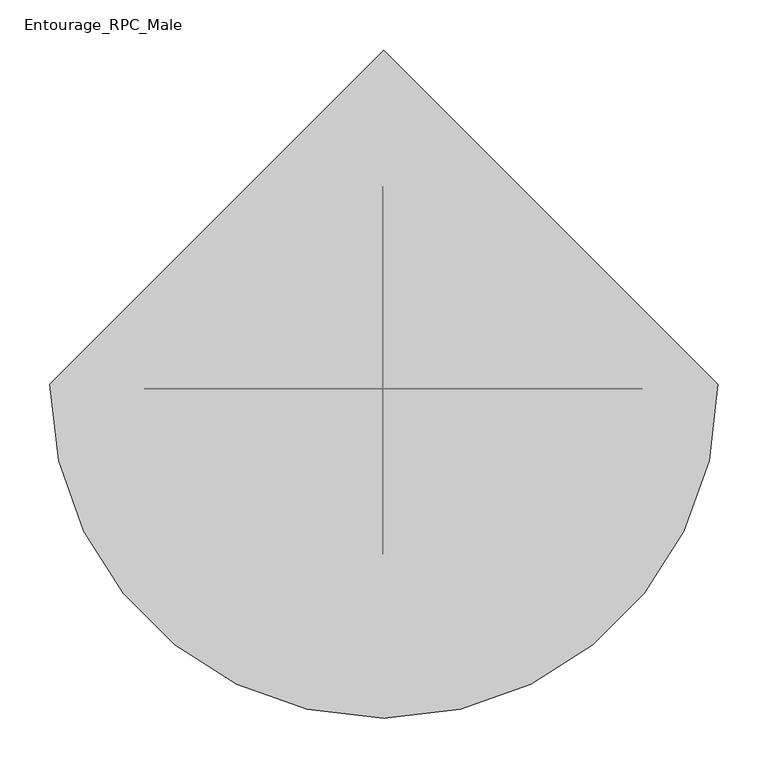
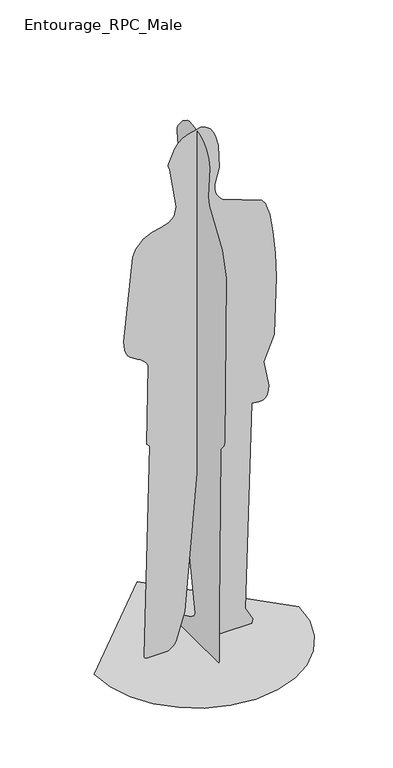
"""IFC4 building model written with IfcOpenShell, lengths in millimetres: proxy geometry, Entourage_RPC_Male : Dwayne."""

from ifc_helpers import new_model, si_unit, origin, place, context, project, spatial, triangles, source, transform, mapped, element, save


def entourage_rpc_male_e00c4429(model_context):
    return source(origin(), model_context, "Body", "Tessellation", [
        triangles([(-180.7519758, -4.45e-05, 5.61e-05), (-184.2427693, -8.8e-06, 2.7953145), (-186.1721755, 1.66e-05, 5.8375002), (-186.8316374, 3.35e-05, 9.127569), (-168.2846227, 8.5e-06, 733.0652109), (-173.8813015, 8.5e-06, 735.2240908), (-177.6698602, 8.1e-06, 740.93319), (-174.1985423, -8.1e-06, 1013.6682867), (-179.591309, -8.8e-06, 1024.1651751), (-188.0395216, -9.6e-06, 1032.7759867), (-198.5267085, -9.9e-06, 1040.1126028), (-210.0363257, -1.03e-05, 1046.7864687), (-221.5520472, -1.07e-05, 1053.4092476), (-232.0572199, -1.1e-05, 1060.5929661), (-240.5353907, -1.14e-05, 1068.9488514), (-245.9518842, -1.21e-05, 1078.9880642), (-249.7386988, -1.29e-05, 1091.9821838), (-252.1552483, -1.4e-05, 1106.9298906), (-253.4607645, -1.47e-05, 1122.8295742), (-224.2188539, -3.16e-05, 1405.054644), (-213.7949444, -3.31e-05, 1430.2019463), (-189.1319694, -3.46e-05, 1456.0842327), (-160.624934, -3.53e-05, 1468.8737137), (-131.9229886, -3.57e-05, 1475.6378357), (-106.6752928, -3.64e-05, 1483.4436092), (-88.5310242, -3.71e-05, 1499.3593529), (-81.1392697, -3.9e-05, 1530.4516411), (-102.942045, -4.71e-05, 1666.4696468), (-107.9472446, -4.78e-05, 1679.2650867), (-108.1474504, -4.82e-05, 1680.5741638), (-107.984815, -4.82e-05, 1682.7587688), (-107.5268306, -4.82e-05, 1685.5190655), (-106.840944, -4.86e-05, 1688.5553627), (-86.6409052, -5.11e-05, 1733.0902897), (-74.2774293, -5.19e-05, 1747.7183212), (-59.5121605, -5.26e-05, 1759.6594528), (-42.363121, -5.33e-05, 1768.7777916), (-0.9855255, -5.37e-05, 1777.9990311), (15.8808757, -5.33e-05, 1772.5528519), (29.1619555, -5.26e-05, 1761.5639877), (39.2640369, -5.19e-05, 1747.0962662), (46.5934632, -5.08e-05, 1731.2140961), (56.009163, -4.89e-05, 1695.7207684), (59.1639487, -4.41e-05, 1618.2087845), (44.4858339, -4.12e-05, 1564.7278919), (44.3096682, -4.05e-05, 1551.1862766), (46.5532813, -3.94e-05, 1537.9279289), (51.2886345, -3.86e-05, 1525.4359589), (58.5876575, -3.83e-05, 1514.1926044), (68.5223164, -3.75e-05, 1504.6808304), (198.4030241, -3.46e-05, 1454.5808361), (210.7095586, -3.38e-05, 1440.8296406), (224.9005892, -3.13e-05, 1397.8447643), (235.5369131, -2.72e-05, 1333.6069702), (242.7580384, -2.28e-05, 1256.1532677), (246.7032373, -1.77e-05, 1173.5211021), (240.2781571, -5.9e-06, 974.9290089), (206.081389, -1.1e-06, 891.6222479), (221.1961823, 4e-06, 805.6633232), (220.4650678, 5.1e-06, 788.6200321), (214.9948893, 6.3e-06, 771.8045614), (210.3552016, 6.6e-06, 765.7300776), (204.1668257, 6.6e-06, 762.0919275), (196.8959759, 7e-06, 760.3982082), (189.0090118, 7e-06, 760.1573799), (180.9721295, 7e-06, 760.8774668), (173.2515615, 6.6e-06, 762.0669291), (166.3135766, 6.6e-06, 763.2339363), (144.8011179, 4.49e-05, 59.4752896), (168.6275342, 4.74e-05, 15.3365843), (166.1985945, -4.45e-05, 5.61e-05), (66.1332089, -4.45e-05, 5.61e-05), (49.8425018, -1.03e-05, 3.9765591), (39.0246256, 1.36e-05, 14.0353), (32.5983009, 2.91e-05, 28.3297116), (-2.7441046, 9.2e-06, 720.0458748), (-54.0725034, 1.03e-05, 117.9433278), (-81.3720135, -2.13e-05, 28.0047427), (-85.5237041, -2.69e-05, 19.9172686), (-91.2433859, -3.27e-05, 12.5691172), (-99.2451413, -3.86e-05, 5.9378887), (-110.2431982, -4.45e-05, 5.61e-05), (-13.8237406, -127.6718764, 9.9621145), (-13.8237974, -127.2617633, 182.0842528), (-13.8237815, -135.2635732, 744.8695776), (-13.8237815, -136.4149928, 748.3460369), (-13.8237815, -139.3954704, 752.5736132), (-13.8237815, -143.4944026, 757.5058702), (-13.8237815, -148.0010861, 763.0962994), (-13.8237815, -152.2049901, 769.2983917), (-13.8237792, -155.3953659, 776.0656385), (-13.8237792, -156.8616281, 783.3516764), (-13.8237622, -165.9465024, 1358.6137287), (-13.8237599, -143.2743216, 1442.0927902), (-13.8237576, -71.1145501, 1552.8585583), (-13.8237576, -64.3401725, 1580.5206779), (-13.8237542, -73.5344014, 1684.7952724), (-13.8237531, -67.2131212, 1712.2161278), (-13.8237531, -55.241223, 1734.9070393), (-13.8237531, -37.9260212, 1752.7537697), (-13.8237531, -15.5748771, 1765.6426632), (-13.8237531, 11.5049084, 1773.4593372), (-13.8237531, 43.0059914, 1776.090136), (-13.8237531, 55.0860226, 1772.9164925), (-13.8237542, 79.7038559, 1756.3218658), (-13.8237554, 107.4896145, 1722.3477768), (-13.8237554, 111.5711695, 1713.01012), (-13.8237554, 112.2229284, 1702.3019073), (-13.8237588, 99.0832235, 1611.9284992), (-13.8237588, 100.6007272, 1597.8206394), (-13.8237599, 96.755177, 1579.0656796), (-13.8237622, 31.1784566, 1488.4592915), (-13.8237735, 125.7984261, 1146.7472277), (-13.8237735, 134.1993577, 1137.675107), (-13.8237747, 184.2799037, 1119.3925747), (-13.8237747, 194.4649651, 1111.9394686), (-13.8237747, 201.1343255, 1100.3801451), (-13.8237769, 203.5508567, 1084.2058416), (-13.8237769, 200.9674025, 1068.9640394), (-13.8237769, 194.2820729, 1055.8707253), (-13.8237769, 184.3928146, 1046.1415226), (-13.8237769, 172.1978105, 1040.992709), (-13.8237769, 158.595007, 1041.6399078), (-13.8237769, 144.48246, 1049.299106), (-13.8237838, 123.0429529, 785.7648285), (-13.823786, 116.906318, 707.2429499), (-13.8237928, 10.2023683, 90.6853168), (-13.823794, 17.983895, 76.1481908), (-13.8237951, 35.4714404, 63.806743), (-13.8238042, 104.5965316, 31.8661463), (-13.8238053, 119.3344402, 20.2173661), (-13.8238076, 122.9915025, 6.7192091), (-13.8238042, 122.0607091, 4.3674998), (-13.8237894, 120.3451706, 2.3141478), (-13.8237724, 119.1853577, 1.4285653), (-13.8237474, 117.8199432, 0.6534771), (-13.8237099, 116.2458387, 5.61e-05), (-13.8237077, -124.501612, 0.0), (-348.4734607, 4.7230039, 0.0001684), (-339.5987117, -72.1961519, 0.0001684), (-314.3237646, -142.8340959, 5.61e-05), (-274.6722241, -205.1669827, 5.61e-05), (-222.6681673, -257.171094, 5.61e-05), (-160.3352533, -296.8225073, 5.61e-05), (-89.6973139, -322.097527, 5.61e-05), (-12.7781649, -330.972276, 5.61e-05), (64.1409886, -322.0975634, 5.61e-05), (134.7789371, -296.8225618, 5.61e-05), (197.1118239, -257.1710577, 5.61e-05), (249.1159897, -205.1670008, 5.61e-05), (288.7673667, -142.8340595, 5.61e-05), (314.0423864, -72.1960974, 0.0001684), (322.9171354, 4.7230331, 0.0001684), (-12.7782239, 340.4182474, 0.0001684)], [[70, 71, 72], [69, 70, 72], [69, 72, 73], [69, 73, 74], [69, 74, 75], [69, 75, 76], [68, 69, 76], [82, 1, 2], [82, 2, 3], [82, 3, 4], [81, 82, 4], [80, 81, 4], [79, 80, 4], [78, 79, 4], [77, 78, 4], [77, 4, 5], [76, 77, 5], [5, 6, 7], [76, 5, 7], [76, 7, 8], [68, 76, 8], [67, 68, 8], [66, 67, 8], [65, 66, 8], [64, 65, 8], [63, 64, 8], [62, 63, 8], [61, 62, 8], [60, 61, 8], [59, 60, 8], [58, 59, 8], [57, 58, 8], [56, 57, 8], [56, 8, 9], [55, 56, 9], [55, 9, 10], [54, 55, 10], [54, 10, 11], [53, 54, 11], [53, 11, 12], [52, 53, 12], [51, 52, 12], [50, 51, 12], [50, 12, 13], [50, 13, 14], [50, 14, 15], [50, 15, 16], [50, 16, 17], [50, 17, 18], [50, 18, 19], [50, 19, 20], [50, 20, 21], [50, 21, 22], [50, 22, 23], [50, 23, 24], [50, 24, 25], [50, 25, 26], [49, 50, 26], [48, 49, 26], [48, 26, 27], [47, 48, 27], [46, 47, 27], [45, 46, 27], [44, 45, 27], [44, 27, 28], [43, 44, 28], [42, 43, 28], [42, 28, 29], [42, 29, 30], [42, 30, 31], [42, 31, 32], [42, 32, 33], [42, 33, 34], [42, 34, 35], [42, 35, 36], [42, 36, 37], [41, 42, 37], [40, 41, 37], [40, 37, 38], [40, 38, 39], [137, 138, 83], [137, 83, 84], [136, 137, 84], [135, 136, 84], [130, 131, 132], [130, 132, 133], [130, 133, 134], [130, 134, 135], [122, 123, 124], [121, 122, 124], [120, 121, 124], [119, 120, 124], [118, 119, 124], [117, 118, 124], [116, 117, 124], [115, 116, 124], [114, 115, 124], [113, 114, 124], [106, 107, 108], [105, 106, 108], [104, 105, 108], [103, 104, 108], [102, 103, 108], [101, 102, 108], [100, 101, 108], [99, 100, 108], [98, 99, 108], [97, 98, 108], [97, 108, 109], [97, 109, 110], [97, 110, 111], [96, 97, 111], [95, 96, 111], [95, 111, 112], [94, 95, 112], [93, 94, 112], [93, 112, 113], [92, 93, 113], [92, 113, 124], [92, 124, 125], [91, 92, 125], [90, 91, 125], [89, 90, 125], [88, 89, 125], [87, 88, 125], [86, 87, 125], [86, 125, 126], [85, 86, 126], [85, 126, 127], [84, 85, 127], [84, 127, 128], [135, 84, 128], [135, 128, 129], [130, 135, 129], [153, 154, 139], [152, 153, 139], [152, 139, 140], [151, 152, 140], [151, 140, 141], [151, 141, 142], [150, 151, 142], [149, 150, 142], [149, 142, 143], [149, 143, 144], [149, 144, 145], [149, 145, 146], [149, 146, 147], [149, 147, 148]], closed=False),
    ])


if __name__ == "__main__":
    model = new_model("IFC4")
    model_context = context("Model", 3, world=origin())
    ifc_project = project(units=[si_unit("LENGTHUNIT", "METRE", prefix="MILLI")], contexts=[model_context])
    site = spatial("IfcSite", under=ifc_project)
    building = spatial("IfcBuilding", under=site)
    placement = place(None, origin())
    entourage_rpc_male_shape = entourage_rpc_male_e00c4429(model_context)
    element("IfcBuildingElementProxy", 1, Name="Entourage_RPC_Male : Dwayne", ObjectType="Entourage_RPC_Male : Dwayne", at=placement, inside=building, context=model_context, shape_type="MappedRepresentation", body=[
        mapped(entourage_rpc_male_shape, transform((0.0, 0.0, 0.0), x_axis=(1.0, 0.0, 0.0), y_axis=(0.0, 1.0, 0.0), z_axis=(0.0, 0.0, 1.0))),
    ])
    save(model, "model.ifc")

# Revit data of these elements
# Type "Entourage_RPC_Male : Dwayne"
#   built-in parameter 1005198 = "{2, 15},{22, RPC-8-G1AE-S4G0-CKUK-A},{1, 0},{1, 0},{2, 15},{1, 8},{5, Color},{1, 0},{1, 0},{3, 0.8},{3, 0.8},{3, 0.8},{1, 8},{7, BBoxMin},{1, 0},{1, 0},{1, 0},{1, 0},{1, 0},{1, 8},{7, BBoxMax},{1, 0},{1, 0},{1, 0},{1, 0},{1, 0},{2, 11},{9, RPCTypeId},{1, 0},{1, 0},{22, RPC-8-G1AE-S4G0-CKUK-A},{1, 6},{14, RPCPlantHeight},{1, 0},{1, 0},{7, 5.83333},{2, 11},{7, keyword},{1, 0},{1, 0},{45, :RPCs:People [Business-Hispanic]:Geometry:RPC},{2, 11},{8, category},{1, 0},{1, 0},{26, People [Business-Hispanic]},{2, 11},{12, LocalizedUID},{1, 0},{1, 0},{6, Dwayne},{2, 14},{6, Height},{1, 0},{1, 0},{7, 5.83333},{1, 2},{16, Cast Reflections},{1, 0},{1, 0},{1, 0},{1, 2},{6, Jitter},{1, 0},{1, 0},{1, 1},{1, 2},{9, Billboard},{1, 0},{1, 0},{1, 0},{1, 2},{12, Cast Shadows},{1, 0},{1, 0},{1, 1},{1, 2},{20, Apply Filter Effects},{1, 0},{1, 0},{1, 0},{2, 11},{28, Apply Filter Effects-Text-FC},{1, 0},{1, 0},{4, None},{21, assetlibrary_base.fbx},{1, 5},"
#   built-in parameter 1005195 = "RPC-8-G1AE-S4G0-CKUK-A"
#   Height = 0
